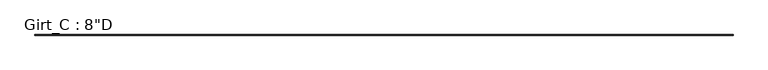
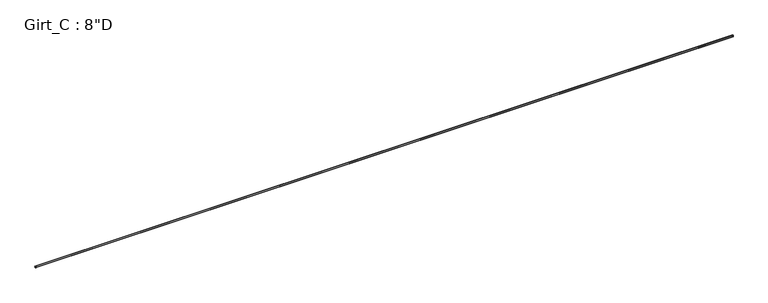
"""IFC4 building model written with IfcOpenShell, lengths in millimetres: beam geometry."""

from ifc_helpers import new_model, si_unit, point, frame, frame_2d, origin, place, context, project, spatial, polyline, circle_curve, trimmed, segment, composite_curve, outline, extrude, source, transform, mapped, element, save


def beam_e6d9bcd1(model_context):
    return source(origin(), model_context, "Body", "SweptSolid", [
        extrude(outline(composite_curve([segment(polyline([(87.5109375, 101.6), (99.7560415, 87.0068534), (97.6278742, 85.221109), (86.2154765, 98.821875), (3.3005807, 98.821875)]), True, "CONTINUOUS"), segment(trimmed(circle_curve(frame_2d((3.3741066, 96.8381931)), 1.9850441), [point((3.3005807, 98.821875))], [point((1.3890625, 96.8381931))], True, "CARTESIAN"), True, "CONTINUOUS"), segment(polyline([(1.3890625, 96.8381931), (1.3890625, -96.8389339)]), True, "CONTINUOUS"), segment(trimmed(circle_curve(frame_2d((3.3748024, -96.8389339)), 1.9857399), [point((1.3890625, -96.8389339))], [point((3.2694106, -98.821875))], True, "CARTESIAN"), True, "CONTINUOUS"), segment(polyline([(3.2694106, -98.821875), (86.2154765, -98.821875), (97.6510975, -85.1934327), (99.7792647, -86.979177), (87.5109375, -101.6), (3.3734375, -101.6)]), True, "CONTINUOUS"), segment(trimmed(circle_curve(frame_2d((3.3734375, -96.8375)), 4.7625), [point((3.3734375, -101.6))], [point((-1.3890625, -96.8375))], False, "CARTESIAN"), True, "CONTINUOUS"), segment(polyline([(-1.3890625, -96.8375), (-1.3890625, 96.8375)]), True, "CONTINUOUS"), segment(trimmed(circle_curve(frame_2d((3.3734375, 96.8375)), 4.7625), [point((-1.3890625, 96.8375))], [point((3.3734375, 101.6))], False, "CARTESIAN"), True, "CONTINUOUS"), segment(polyline([(3.3734375, 101.6), (87.5109375, 101.6)]), True, "CONTINUOUS")], self_intersect=False)), frame((-53349.3086819, 0.0, 0.0), z_axis=(1.0, 0.0, 0.0), x_axis=(0.0, 1.0, 0.0)), (0.0, 0.0, 1.0), 106698.6173639),
    ])


if __name__ == "__main__":
    model = new_model("IFC4")
    model_context = context("Model", 3, world=origin())
    ifc_project = project(units=[si_unit("LENGTHUNIT", "METRE", prefix="MILLI")], contexts=[model_context])
    site = spatial("IfcSite", under=ifc_project)
    building = spatial("IfcBuilding", under=site)
    placement = place(None, origin())
    beam_shape = beam_e6d9bcd1(model_context)
    element("IfcBeam", 1, ObjectType="Girt_C : 8\"D", at=placement, inside=building, context=model_context, shape_type="MappedRepresentation", body=[
        mapped(beam_shape, transform((0.0, 0.0, 0.0), x_axis=(1.0, 0.0, 0.0), y_axis=(0.0, 1.0, 0.0), z_axis=(0.0, 0.0, 1.0))),
    ])
    save(model, "model.ifc")

# Revit data of these elements
# Type "Girt_C : 8\"D"
#   half leg = 0' - 1 3/4"
#   Web_Thickness = 0' - 0 7/64"
#   Length [instance default] = 10' - 0"
#   Leg_1 = 0' - 3 1/2"
#   Height = 0' - 8"
#   Structural Material [instance default] = none
# Element 1 (IfcBeam, "Girt_C : 8\"D")
#   Structural Material = CEE' SECTION (8.0x3.5C - SEE STRUCT. DWGS)
#   Materials on its faces: "CEE' SECTION (8.0x3.5C - SEE STRUCT. DWGS)"
# Materials
#   "CEE' SECTION (8.0x3.5C - SEE STRUCT. DWGS)": class "Metal", colour RGB 137 146 153, transparency 0, Description = "Steel, mill finish", Cost = 0
